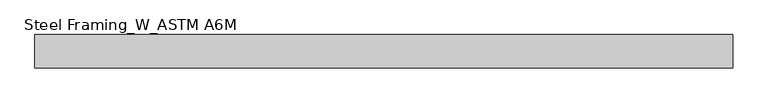
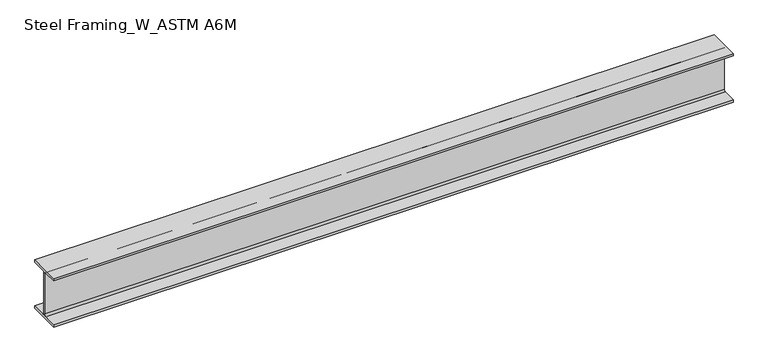
"""IFC4 building model written with IfcOpenShell, lengths in millimetres: beam geometry, Steel Framing_W_ASTM A6M : H_SB_AR_S02_W200x31.3_B6."""

from ifc_helpers import new_model, si_unit, point, frame, frame_2d, origin, place, context, project, spatial, polyline, circle_curve, trimmed, segment, composite_curve, outline, extrude, source, transform, mapped, element, save


def steel_framing_w_astm_a6m_0a69f8b6(model_context):
    return source(origin(), model_context, "Body", "SweptSolid", [
        extrude(outline(composite_curve([segment(polyline([(67.0, -94.8), (67.0, -105.0), (-67.0, -105.0), (-67.0, -94.8), (-10.775, -94.8)]), True, "CONTINUOUS"), segment(trimmed(circle_curve(frame_2d((-10.775, -87.2)), 7.6), [point((-10.775, -94.8))], [point((-3.175, -87.2))], True, "CARTESIAN"), True, "CONTINUOUS"), segment(polyline([(-3.175, -87.2), (-3.175, 87.2)]), True, "CONTINUOUS"), segment(trimmed(circle_curve(frame_2d((-10.775, 87.2)), 7.6), [point((-3.175, 87.2))], [point((-10.775, 94.8))], True, "CARTESIAN"), True, "CONTINUOUS"), segment(polyline([(-10.775, 94.8), (-67.0, 94.8), (-67.0, 105.0), (67.0, 105.0), (67.0, 94.8), (10.775, 94.8)]), True, "CONTINUOUS"), segment(trimmed(circle_curve(frame_2d((10.775, 87.2)), 7.6), [point((10.775, 94.8))], [point((3.175, 87.2))], True, "CARTESIAN"), True, "CONTINUOUS"), segment(polyline([(3.175, 87.2), (3.175, -87.2)]), True, "CONTINUOUS"), segment(trimmed(circle_curve(frame_2d((10.775, -87.2)), 7.6), [point((3.175, -87.2))], [point((10.775, -94.8))], True, "CARTESIAN"), True, "CONTINUOUS"), segment(polyline([(10.775, -94.8), (67.0, -94.8)]), True, "CONTINUOUS")], self_intersect=False)), frame((-1385.8, 0.0, 0.0), z_axis=(1.0, 0.0, 0.0), x_axis=(0.0, 1.0, 0.0)), (0.0, 0.0, 1.0), 2787.6),
    ])


if __name__ == "__main__":
    model = new_model("IFC4")
    model_context = context("Model", 3, world=origin())
    ifc_project = project(units=[si_unit("LENGTHUNIT", "METRE", prefix="MILLI")], contexts=[model_context])
    site = spatial("IfcSite", under=ifc_project)
    building = spatial("IfcBuilding", under=site)
    placement = place(None, origin())
    steel_framing_w_astm_a6m_shape = steel_framing_w_astm_a6m_0a69f8b6(model_context)
    element("IfcBeam", 1, ObjectType="Steel Framing_W_ASTM A6M : H_SB_AR_S02_W200x31.3_B6", at=placement, inside=building, context=model_context, shape_type="MappedRepresentation", body=[
        mapped(steel_framing_w_astm_a6m_shape, transform((0.0, 0.0, 0.0), x_axis=(1.0, 0.0, 0.0), y_axis=(0.0, 1.0, 0.0), z_axis=(0.0, 0.0, 1.0))),
    ])
    save(model, "model.ifc")

# Revit data of these elements
# Project information
#   Project Status = "Project Status"
#   Client Name = "현대엔지니어링"
#   Project Address = "서울시 종로구 율곡로 75(계동)"
#   Project Number = "-"
# Type "Steel Framing_W_ASTM A6M : H_SB_AR_S02_W200x31.3_B6"
#   Type Mark = "B6"
#   Section Name Key = "W8x21"
#   Width = 13.4 cm
#   Web Thickness = 0.635 cm
#   Web Fillet = 0.76 cm
#   Warping Constant = 40800.0 cm⁶
#   Torsional Moment of Inertia = 11.70 cm⁴
#   Section Area = 39.7 cm²
#   Plastic Modulus weak axis = 93.2 cm³
#   Plastic Modulus strong axis = 334.0 cm³
#   Perimeter = 0.93 m²/m
#   Nominal Weight = 31.30 kgf/m
#   Moment of Inertia weak axis = 407.00 cm⁴
#   Moment of Inertia strong axis = 3130.00 cm⁴
#   Height = 21.0 cm
#   Flange Thickness = 1.02 cm
#   Elastic Modulus weak axis = 60.8 cm³
#   Elastic Modulus strong axis = 298.0 cm³
#   Centroid Vertical = 10.5 cm
#   Centroid Horizontal = 6.7 cm
#   Length [instance default] = 1500 mm
#   Structural Material [instance default] = Steel, 45-345
#   Bolt Spacing = 0
#   Assembly Code = ""
# Element 1 (IfcBeam, "Steel Framing_W_ASTM A6M : H_SB_AR_S02_W200x31.3_B6")
#   Materials on its faces: "Steel, 45-345"
# Materials
#   "Steel, 45-345": class "Metal", colour RGB 189 187 185, transparency 0, Description = "Steel 345 MPa", Cost = 0
